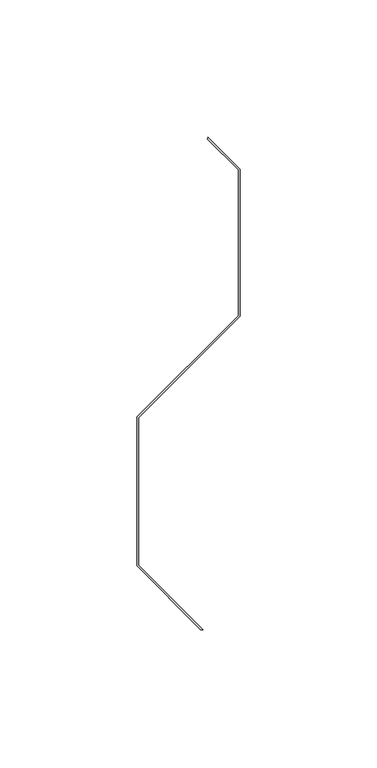
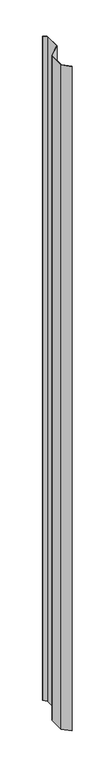
"""IFC4 building model written with IfcOpenShell, lengths in millimetres: proxy geometry, MBCI 7.2-V Panel9 : MBCI 7.2-V Panel-1."""

from ifc_helpers import new_model, si_unit, frame, origin, place, context, project, spatial, polyline, outline, extrude, source, transform, mapped, element, save


def generic_models_5dc78b0a(model_context):
    return source(origin(), model_context, "Body", "SweptSolid", [
        extrude(outline(polyline([(587365.2695864, -535087.4383203), (587328.3744989, -535124.3334078), (587328.3744989, -535178.1208986), (587351.8199844, -535201.5663841), (587350.9780854, -535201.5663841), (587327.7791864, -535178.3674851), (587327.7791864, -535124.0868213), (587364.6742739, -535087.1917338), (587364.6742739, -535034.1036068), (587353.54384, -535022.9731729), (587353.5988637, -535022.1862976), (587365.2695864, -535033.8570203), (587365.2695864, -535087.4383203)])), frame((0.0, 0.0, 51.59375), z_axis=(0.0, 0.0, 1.0), x_axis=(1.0, 0.0, 0.0)), (0.0, 0.0, 1.0), 2386.80625),
    ])


if __name__ == "__main__":
    model = new_model("IFC4")
    model_context = context("Model", 3, world=origin())
    ifc_project = project(units=[si_unit("LENGTHUNIT", "METRE", prefix="MILLI")], contexts=[model_context])
    site = spatial("IfcSite", under=ifc_project)
    building = spatial("IfcBuilding", under=site)
    placement = place(None, origin())
    generic_models_shape = generic_models_5dc78b0a(model_context)
    element("IfcBuildingElementProxy", 1, Name="MBCI 7.2-V Panel9 : MBCI 7.2-V Panel-1", ObjectType="MBCI 7.2-V Panel9 : MBCI 7.2-V Panel-1", at=placement, inside=building, context=model_context, shape_type="MappedRepresentation", body=[
        mapped(generic_models_shape, transform((0.0, 0.0, 0.0), x_axis=(1.0, 0.0, 0.0), y_axis=(0.0, 1.0, 0.0), z_axis=(0.0, 0.0, 1.0))),
    ])
    save(model, "model.ifc")

# Revit data of these elements
# Element 1 (IfcBuildingElementProxy, "MBCI 7.2-V Panel9 : MBCI 7.2-V Panel-1")
#   Materials on its faces: "MTL PANEL"
# Materials
#   "MTL PANEL": class "Generic", colour RGB 239 242 240, transparency 0, Cost = 0
